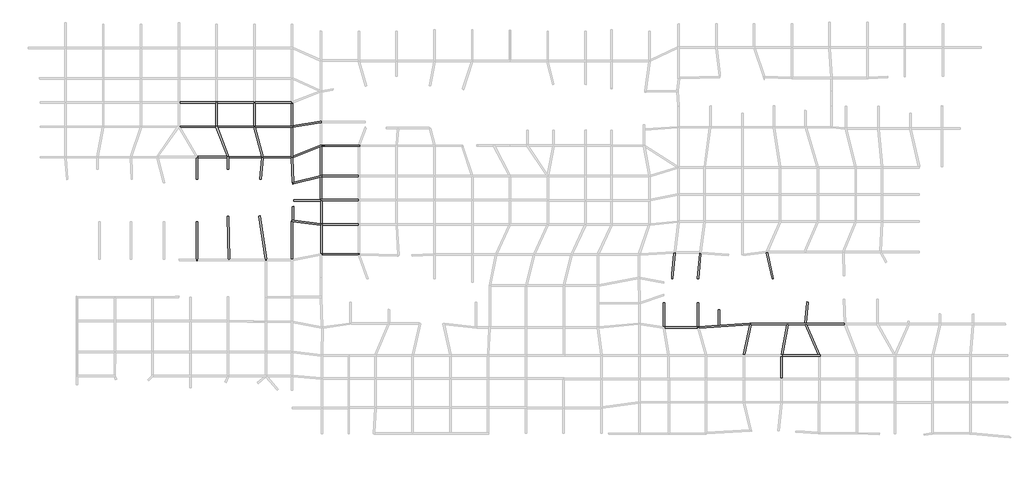
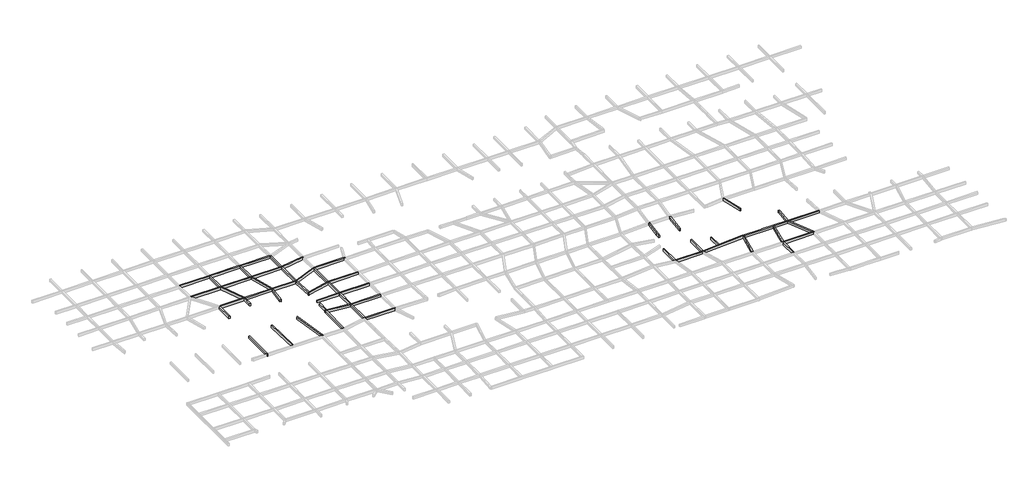
# One storey, part 6 of 15: 53 beams.
"""IFC4 building model written with IfcOpenShell, lengths in millimetres."""

from ifc_helpers import new_model, si_unit, frame, origin, place, context, project, spatial, polyline, outline, extrude, faceted_brep, element, save

model = new_model("IFC4")

# Units and contexts
model_context = context("Model", 3, world=origin())
ifc_project = project(units=[si_unit("LENGTHUNIT", "METRE", prefix="MILLI")], contexts=[model_context])

# Site, building, storey
site = spatial("IfcSite", under=ifc_project)
building = spatial("IfcBuilding", under=site)
storey = spatial("IfcBuildingStorey", under=building, Name="层高", Elevation=3300.0)

# Beams
placement = place(None, origin())
element("IfcBeam", 1, ObjectType="混凝土 - 矩形梁 : KL_beam", at=placement, inside=storey, context=model_context, shape_type="Brep", body=[
    faceted_brep([(153850.3013477, 63968.1790994, 3300.0), (153925.2394262, 63982.5367156, 3300.0), (153925.2394262, 64256.5260367, 3300.0), (153925.2394262, 70092.1684205, 3300.0), (153925.2394262, 70392.1684205, 3300.0), (153625.2394262, 70392.1684205, 3300.0), (153625.2394262, 70122.3059852, 3300.0), (153625.2394262, 64230.5153579, 3300.0), (153793.8501921, 64262.8200114, 3300.0), (153625.2394262, 64230.5153579, 2700.0), (153625.2394262, 70392.1684205, 2700.0), (153625.2394262, 70122.3059852, 2700.0), (153925.2394262, 63982.5367156, 2700.0), (153850.3013477, 63968.1790994, 2700.0), (153793.8501921, 64262.8200114, 2700.0), (153925.2394262, 70392.1684205, 2700.0), (153925.2394262, 70092.1684205, 2700.0), (153925.2394262, 64256.5260367, 2700.0)], [[[0, 1, 2, 3, 4, 5, 6, 7, 8]], [[9, 7, 6, 5, 10, 11]], [[12, 13, 14, 9, 11, 10, 15, 16, 17]], [[1, 12, 17, 16, 15, 4, 3, 2]], [[12, 1, 0, 13]], [[14, 8, 7, 9]], [[8, 14, 13, 0]], [[5, 4, 15, 10]]]),
])
element("IfcBeam", 2, ObjectType="混凝土 - 矩形梁 : KL_beam", at=placement, inside=storey, context=model_context, shape_type="Brep", body=[
    faceted_brep([(153925.2394262, 64256.5260367, 2700.0), (153925.2394262, 64256.5260367, 3300.0), (161350.300938, 64256.5260367, 3300.0), (161650.300938, 64256.5260367, 3300.0), (161650.300938, 64256.5260367, 2700.0), (161350.300938, 64256.5260367, 2700.0), (153925.2394262, 63982.5367156, 2700.0), (153925.2394262, 63982.5367156, 3300.0), (153850.3013477, 63968.1790994, 2700.0), (153850.3013477, 63968.1790994, 3300.0), (153850.3013477, 63956.5260367, 3300.0), (161393.3069779, 63956.5260367, 3300.0), (161497.8826169, 63956.5260367, 3300.0), (161650.300938, 63956.5260367, 3300.0), (161650.300938, 64251.7661343, 3300.0), (161650.300938, 63956.5260367, 2700.0), (153850.3013477, 63956.5260367, 2700.0), (161393.3069779, 63956.5260367, 2700.0), (161497.8826169, 63956.5260367, 2700.0), (161650.300938, 64251.7661343, 2700.0)], [[[0, 1, 2, 3, 4, 5]], [[6, 7, 1, 0]], [[7, 6, 8, 9]], [[1, 7, 9, 10, 11, 12, 13, 14, 3, 2]], [[15, 13, 12, 11, 10, 16, 17, 18]], [[6, 0, 5, 4, 19, 15, 18, 17, 16, 8]], [[9, 8, 16, 10]], [[3, 14, 13, 15, 19, 4]]]),
])
element("IfcBeam", 3, ObjectType="混凝土 - 矩形梁 : KL_beam", at=placement, inside=storey, context=model_context, shape_type="SweptSolid", body=[
    extrude(outline(polyline([(153925.2394262, 70092.1684205), (153925.2394262, 70392.1684205), (161350.300938, 70392.1684205), (161350.300938, 70092.1684205), (153925.2394262, 70092.1684205)])), frame((0.0, 0.0, 2700.0), z_axis=(0.0, 0.0, 1.0), x_axis=(1.0, 0.0, 0.0)), (0.0, 0.0, 1.0), 600.0),
])
element("IfcBeam", 4, ObjectType="混凝土 - 矩形梁 : KL_beam", at=placement, inside=storey, context=model_context, shape_type="Brep", body=[
    faceted_brep([(248649.8189959, 38517.26105, 3300.0), (248949.8189959, 38517.26105, 3300.0), (248949.8189959, 38542.26105, 3300.0), (248949.8189959, 43042.26105, 3300.0), (248649.8189959, 43042.26105, 3300.0), (248949.8189959, 38517.26105, 2700.0), (248949.8189959, 38542.26105, 2700.0), (248949.8189959, 43042.26105, 2700.0), (248649.8189959, 38517.26105, 2700.0), (248649.8189959, 43042.26105, 2700.0)], [[[0, 1, 2, 3, 4]], [[1, 5, 6, 7, 3, 2]], [[5, 8, 9, 7, 6]], [[8, 0, 4, 9]], [[1, 0, 8, 5]], [[4, 3, 7, 9]]]),
])
element("IfcBeam", 5, ObjectType="混凝土 - 矩形梁 : KL_beam", at=placement, inside=storey, context=model_context, shape_type="Brep", body=[
    faceted_brep([(256749.8189959, 43042.26105, 3300.0), (256749.8189959, 43342.26105, 3300.0), (256698.3032407, 43342.26105, 3300.0), (256371.3560571, 43342.26105, 3300.0), (248981.7835465, 43342.26105, 3300.0), (248949.8189959, 43342.26105, 3300.0), (248949.8189959, 43042.26105, 3300.0), (256449.8189959, 43042.26105, 3300.0), (256749.8189959, 43042.26105, 2700.0), (248949.8189959, 43042.26105, 2700.0), (256449.8189959, 43042.26105, 2700.0), (256749.8189959, 43342.26105, 2700.0), (248949.8189959, 43342.26105, 2700.0), (248981.7835465, 43342.26105, 2700.0), (256371.3560571, 43342.26105, 2700.0), (256698.3032407, 43342.26105, 2700.0)], [[[0, 1, 2, 3, 4, 5, 6, 7]], [[8, 0, 7, 6, 9, 10]], [[11, 8, 10, 9, 12, 13, 14, 15]], [[1, 11, 15, 14, 13, 12, 5, 4, 3, 2]], [[6, 5, 12, 9]], [[1, 0, 8, 11]]]),
])
element("IfcBeam", 6, ObjectType="混凝土 - 矩形梁 : KL_beam", at=placement, inside=storey, context=model_context, shape_type="Brep", body=[
    faceted_brep([(261774.3457024, 49601.7141002, 3300.0), (261774.3457024, 49901.7141002, 3300.0), (261720.5296547, 49901.7141002, 3300.0), (253919.7116815, 49901.7141002, 3300.0), (253618.8431569, 49901.7141002, 3300.0), (247159.7341687, 49901.7141002, 3300.0), (247159.7341687, 49841.7141002, 3300.0), (247039.7341687, 49841.7141002, 3300.0), (242265.632488, 49841.7141002, 3300.0), (242214.4093203, 49601.7141002, 3300.0), (242521.1660768, 49601.7141002, 3300.0), (249892.882957, 49601.7141002, 3300.0), (250198.4979655, 49601.7141002, 3300.0), (253659.3709471, 49601.7141002, 3300.0), (253986.3181308, 49601.7141002, 3300.0), (261774.3457024, 49901.7141002, 2700.0), (261774.3457024, 49601.7141002, 2700.0), (253986.3181308, 49601.7141002, 2700.0), (253659.3709471, 49601.7141002, 2700.0), (250198.4979655, 49601.7141002, 2700.0), (249892.882957, 49601.7141002, 2700.0), (242521.1660768, 49601.7141002, 2700.0), (242214.4093203, 49601.7141002, 2700.0), (242265.632488, 49841.7141002, 2700.0), (247159.7341687, 49841.7141002, 2700.0), (247159.7341687, 49901.7141002, 2700.0), (253618.8431569, 49901.7141002, 2700.0), (253919.7116815, 49901.7141002, 2700.0), (261720.5296547, 49901.7141002, 2700.0)], [[[0, 1, 2, 3, 4, 5, 6, 7, 8, 9, 10, 11, 12, 13, 14]], [[15, 16, 17, 18, 19, 20, 21, 22, 23, 24, 25, 26, 27, 28]], [[16, 0, 14, 13, 12, 11, 10, 9, 22, 21, 20, 19, 18, 17]], [[1, 0, 16, 15]], [[22, 9, 8, 23]], [[24, 6, 5, 25]], [[6, 24, 23, 8, 7]], [[1, 15, 28, 27, 26, 25, 5, 4, 3, 2]]]),
])
element("IfcBeam", 7, ObjectType="混凝土 - 矩形梁 : KL_beam", at=placement, inside=storey, context=model_context, shape_type="Brep", body=[
    faceted_brep([(256371.3560571, 43342.26105, 2700.0), (256371.3560571, 43342.26105, 3300.0), (253659.3709471, 49601.7141002, 3300.0), (253659.3709471, 49601.7141002, 2700.0), (256449.8189959, 43342.26105, 2700.0), (256698.3032407, 43342.26105, 2700.0), (256698.3032407, 43342.26105, 3300.0), (256449.8189959, 43342.26105, 3300.0), (253986.3181308, 49601.7141002, 3300.0), (253986.3181308, 49601.7141002, 2700.0)], [[[0, 1, 2, 3]], [[1, 0, 4, 5, 6, 7]], [[7, 6, 8, 2, 1]], [[4, 0, 3, 9, 5]], [[6, 5, 9, 8]], [[3, 2, 8, 9]]]),
])
element("IfcBeam", 8, ObjectType="混凝土 - 矩形梁 : KL_beam", at=placement, inside=storey, context=model_context, shape_type="Brep", body=[
    faceted_brep([(248676.168538, 43342.26105, 3300.0), (248949.8189959, 43342.26105, 3300.0), (248981.7835465, 43342.26105, 3300.0), (250198.4979655, 49601.7141002, 3300.0), (249892.882957, 49601.7141002, 3300.0), (248981.7835465, 43342.26105, 2700.0), (250198.4979655, 49601.7141002, 2700.0), (248949.8189959, 43342.26105, 2700.0), (248676.168538, 43342.26105, 2700.0), (249892.882957, 49601.7141002, 2700.0)], [[[0, 1, 2, 3, 4]], [[2, 5, 6, 3]], [[5, 7, 8, 9, 6]], [[8, 0, 4, 9]], [[0, 8, 7, 5, 2, 1]], [[4, 3, 6, 9]]]),
])
element("IfcBeam", 9, ObjectType="混凝土 - 矩形梁 : KL_beam", at=placement, inside=storey, context=model_context, shape_type="Brep", body=[
    faceted_brep([(253950.2144032, 54253.3773688, 2700.0), (253950.2144032, 54253.3773688, 3300.0), (253964.038385, 54252.3246977, 3300.0), (253964.038385, 54252.3246977, 2700.0), (253950.1342442, 54252.3246977, 2700.0), (253950.1342442, 54252.3246977, 3300.0)], [[[0, 1, 2, 3]], [[0, 3, 4]], [[3, 2, 5, 4]], [[2, 1, 5]], [[1, 0, 4, 5]]]),
    faceted_brep([(253919.7116815, 49901.7141002, 3300.0), (254249.3483857, 54230.5988599, 3300.0), (254109.7167317, 54241.2315565, 3300.0), (254109.7167317, 54132.3246977, 3300.0), (253989.7167317, 54132.3246977, 3300.0), (253940.9964624, 54132.3246977, 3300.0), (253618.8431569, 49901.7141002, 3300.0), (253618.8431569, 49901.7141002, 2700.0), (253940.9964624, 54132.3246977, 2700.0), (254249.3483857, 54230.5988599, 2700.0), (253919.7116815, 49901.7141002, 2700.0), (254109.7167317, 54132.3246977, 2700.0), (254109.7167317, 54241.2315565, 2700.0)], [[[0, 1, 2, 3, 4, 5, 6]], [[7, 6, 5, 8]], [[9, 1, 0, 10]], [[0, 6, 7, 10]], [[11, 3, 2, 12]], [[3, 11, 8, 5, 4]], [[1, 9, 12, 2]], [[9, 10, 7, 8, 11, 12]]]),
])
element("IfcBeam", 10, ObjectType="混凝土 - 矩形梁 : KL_beam", at=placement, inside=storey, context=model_context, shape_type="Brep", body=[
    faceted_brep([(240878.4550975, 43342.26105, 3300.0), (241149.8189959, 43342.26105, 3300.0), (241185.211854, 43342.26105, 3300.0), (242521.1660768, 49601.7141002, 3300.0), (242214.4093203, 49601.7141002, 3300.0), (242211.3807699, 49587.5241911, 3300.0), (241185.211854, 43342.26105, 2700.0), (242521.1660768, 49601.7141002, 2700.0), (241149.8189959, 43342.26105, 2700.0), (240878.4550975, 43342.26105, 2700.0), (242211.3807699, 49587.5241911, 2700.0), (242214.4093203, 49601.7141002, 2700.0)], [[[0, 1, 2, 3, 4, 5]], [[2, 6, 7, 3]], [[6, 8, 9, 10, 11, 7]], [[9, 0, 5, 4, 11, 10]], [[0, 9, 8, 6, 2, 1]], [[4, 3, 7, 11]]]),
])
element("IfcBeam", 11, ObjectType="混凝土 - 矩形梁 : KL_beam", at=placement, inside=storey, context=model_context, shape_type="Brep", body=[
    faceted_brep([(231696.6703608, 48978.5566033, 3300.0), (231696.6703608, 49107.4754781, 3300.0), (231541.189145, 49107.4754781, 3300.0), (231396.6703608, 49107.4754781, 3300.0), (224676.6602363, 49107.4754781, 3300.0), (224538.2100932, 49107.4754781, 3300.0), (224676.6602363, 49086.0272569, 3300.0), (224676.6602363, 48969.2807341, 3300.0), (224702.2876712, 48807.4754781, 3300.0), (231433.6372532, 48807.4754781, 3300.0), (231396.6703608, 48936.3943529, 3300.0), (231433.6372532, 48807.4754781, 2700.0), (224702.2876712, 48807.4754781, 2700.0), (231696.6703608, 49107.4754781, 2700.0), (231696.6703608, 48978.5566033, 2700.0), (231396.6703608, 48936.3943529, 2700.0), (224676.6602363, 48969.2807341, 2700.0), (224676.6602363, 49086.0272569, 2700.0), (224538.2100932, 49107.4754781, 2700.0), (224676.6602363, 49107.4754781, 2700.0), (231396.6703608, 49107.4754781, 2700.0), (231541.189145, 49107.4754781, 2700.0)], [[[0, 1, 2, 3, 4, 5, 6, 7, 8, 9, 10]], [[11, 9, 8, 12]], [[13, 14, 15, 11, 12, 16, 17, 18, 19, 20, 21]], [[1, 13, 21, 20, 19, 18, 5, 4, 3, 2]], [[1, 0, 14, 13]], [[10, 9, 11, 15]], [[8, 7, 16, 12]], [[10, 15, 14, 0]], [[17, 6, 5, 18]], [[6, 17, 16, 7]]]),
])
element("IfcBeam", 12, ObjectType="混凝土 - 矩形梁 : KL_beam", at=placement, inside=storey, context=model_context, shape_type="Brep", body=[
    faceted_brep([(231741.7485438, 48821.3502966, 3300.0), (242211.3807699, 49587.5241911, 3300.0), (242214.4093203, 49601.7141002, 3300.0), (242265.632488, 49841.7141002, 3300.0), (242218.4382799, 49841.7141002, 3300.0), (242218.4382799, 49888.8429011, 3300.0), (236049.8021786, 49437.4184534, 3300.0), (235749.8021786, 49415.4642755, 3300.0), (231696.6703608, 49118.8536857, 3300.0), (231541.189145, 49107.4754781, 3300.0), (231696.6703608, 49107.4754781, 3300.0), (231696.6703608, 48978.5566033, 3300.0), (242211.3807699, 49587.5241911, 2700.0), (231741.7485438, 48821.3502966, 2700.0), (231696.6703608, 48978.5566033, 2700.0), (231696.6703608, 49107.4754781, 2700.0), (231541.189145, 49107.4754781, 2700.0), (231696.6703608, 49118.8536857, 2700.0), (235749.8021786, 49415.4642755, 2700.0), (236049.8021786, 49437.4184534, 2700.0), (242218.4382799, 49888.8429011, 2700.0), (242218.4382799, 49841.7141002, 2700.0), (242265.632488, 49841.7141002, 2700.0), (242214.4093203, 49601.7141002, 2700.0)], [[[0, 1, 2, 3, 4, 5, 6, 7, 8, 9, 10, 11]], [[12, 1, 0, 13]], [[12, 13, 14, 15, 16, 17, 18, 19, 20, 21, 22, 23]], [[16, 9, 8, 7, 6, 5, 20, 19, 18, 17]], [[1, 12, 23, 22, 3, 2]], [[0, 11, 14, 13]], [[15, 10, 9, 16]], [[10, 15, 14, 11]], [[21, 4, 3, 22]], [[4, 21, 20, 5]]]),
])
element("IfcBeam", 13, ObjectType="混凝土 - 矩形梁 : KL_beam", at=placement, inside=storey, context=model_context, shape_type="SweptSolid", body=[
    extrude(outline(polyline([(236049.8021786, 49437.4184534), (235749.8021786, 49415.4642755), (235749.8021786, 52693.0860808), (236049.8021786, 52693.0860808), (236049.8021786, 49437.4184534)])), frame((0.0, 0.0, 2700.0), z_axis=(0.0, 0.0, 1.0), x_axis=(1.0, 0.0, 0.0)), (0.0, 0.0, 1.0), 600.0),
])
element("IfcBeam", 14, ObjectType="混凝土 - 矩形梁 : KL_beam", at=placement, inside=storey, context=model_context, shape_type="SweptSolid", body=[
    extrude(outline(polyline([(231541.189145, 49107.4754781), (231396.6703608, 49107.4754781), (231396.6703608, 54132.3246977), (231696.6703608, 54132.3246977), (231696.6703608, 49118.8536857), (231541.189145, 49107.4754781)])), frame((0.0, 0.0, 2700.0), z_axis=(0.0, 0.0, 1.0), x_axis=(1.0, 0.0, 0.0)), (0.0, 0.0, 1.0), 600.0),
])
element("IfcBeam", 15, ObjectType="混凝土 - 矩形梁 : KL_beam", at=placement, inside=storey, context=model_context, shape_type="SweptSolid", body=[
    extrude(outline(polyline([(224376.6602363, 54091.8381482), (224676.6602363, 54091.8381482), (224676.6602363, 49107.4754781), (224538.2100932, 49107.4754781), (224376.6602363, 49132.5022277), (224376.6602363, 54091.8381482)])), frame((0.0, 0.0, 2700.0), z_axis=(0.0, 0.0, 1.0), x_axis=(1.0, 0.0, 0.0)), (0.0, 0.0, 1.0), 600.0),
])
element("IfcBeam", 16, ObjectType="混凝土 - 矩形梁 : KL_beam", at=placement, inside=storey, context=model_context, shape_type="Brep", body=[
    faceted_brep([(153625.2394262, 75445.2581831, 3300.0), (153625.2394262, 75145.2581831, 3300.0), (153925.2394262, 75145.2581831, 3300.0), (161350.300938, 75145.2581831, 3300.0), (161350.300938, 75445.2581831, 3300.0), (153850.3009381, 75445.2581831, 3300.0), (153625.2394262, 75445.2581831, 2700.0), (161350.300938, 75445.2581831, 2700.0), (153850.3009381, 75445.2581831, 2700.0), (153625.2394262, 75145.2581831, 2700.0), (161350.300938, 75145.2581831, 2700.0), (153925.2394262, 75145.2581831, 2700.0)], [[[0, 1, 2, 3, 4, 5]], [[6, 0, 5, 4, 7, 8]], [[9, 6, 8, 7, 10, 11]], [[1, 9, 11, 10, 3, 2]], [[4, 3, 10, 7]], [[1, 0, 6, 9]]]),
])
element("IfcBeam", 17, ObjectType="混凝土 - 矩形梁 : KL_beam", at=placement, inside=storey, context=model_context, shape_type="Brep", body=[
    faceted_brep([(153625.2394262, 70392.1684205, 3300.0), (153925.2394262, 70392.1684205, 3300.0), (153925.2394262, 75145.2581831, 3300.0), (153625.2394262, 75145.2581831, 3300.0), (153625.2394262, 75142.8652747, 3300.0), (153625.2394262, 75102.1202767, 3300.0), (153625.2394262, 70424.6220705, 3300.0), (153925.2394262, 70392.1684205, 2700.0), (153925.2394262, 75145.2581831, 2700.0), (153625.2394262, 70392.1684205, 2700.0), (153625.2394262, 70424.6220705, 2700.0), (153625.2394262, 75102.1202767, 2700.0), (153625.2394262, 75142.8652747, 2700.0), (153625.2394262, 75145.2581831, 2700.0)], [[[0, 1, 2, 3, 4, 5, 6]], [[1, 7, 8, 2]], [[7, 9, 10, 11, 12, 13, 8]], [[9, 0, 6, 5, 4, 3, 13, 12, 11, 10]], [[1, 0, 9, 7]], [[3, 2, 8, 13]]]),
])
element("IfcBeam", 18, ObjectType="混凝土 - 矩形梁 : KL_beam", at=placement, inside=storey, context=model_context, shape_type="Brep", body=[
    faceted_brep([(139785.4057415, 90592.3894162, 3300.0), (139785.4057415, 90292.3894162, 3300.0), (140096.1315792, 90292.3894162, 3300.0), (147550.2032763, 90292.3894162, 3300.0), (147850.2032763, 90292.3894162, 3300.0), (147850.2032763, 90315.315406, 3300.0), (147850.2032763, 90592.3894162, 3300.0), (147687.7917965, 90592.3894162, 3300.0), (147550.2032763, 90592.3894162, 3300.0), (140050.3009381, 90592.3894162, 3300.0), (139785.4057415, 90292.3894162, 2700.0), (140096.1315792, 90292.3894162, 2700.0), (147550.2032763, 90292.3894162, 2700.0), (147850.2032763, 90292.3894162, 2700.0), (139785.4057415, 90592.3894162, 2700.0), (140050.3009381, 90592.3894162, 2700.0), (147550.2032763, 90592.3894162, 2700.0), (147687.7917965, 90592.3894162, 2700.0), (147850.2032763, 90592.3894162, 2700.0), (147850.2032763, 90315.315406, 2700.0)], [[[0, 1, 2, 3, 4, 5, 6, 7, 8, 9]], [[1, 10, 11, 12, 13, 4, 3, 2]], [[10, 14, 15, 16, 17, 18, 19, 13, 12, 11]], [[14, 0, 9, 8, 7, 6, 18, 17, 16, 15]], [[6, 5, 4, 13, 19, 18]], [[0, 14, 10, 1]]]),
])
element("IfcBeam", 19, ObjectType="混凝土 - 矩形梁 : KL_beam", at=placement, inside=storey, context=model_context, shape_type="Brep", body=[
    faceted_brep([(147550.2032763, 84040.4584193, 3300.0), (147850.2032763, 84040.4584193, 3300.0), (147850.2032763, 84363.1269806, 3300.0), (147850.2032763, 90292.3894162, 3300.0), (147550.2032763, 90292.3894162, 3300.0), (147550.2032763, 84292.3894162, 3300.0), (147550.2032763, 84040.4584193, 2700.0), (147550.2032763, 90292.3894162, 2700.0), (147550.2032763, 84292.3894162, 2700.0), (147850.2032763, 84040.4584193, 2700.0), (147850.2032763, 90292.3894162, 2700.0), (147850.2032763, 84363.1269806, 2700.0)], [[[0, 1, 2, 3, 4, 5]], [[6, 0, 5, 4, 7, 8]], [[9, 6, 8, 7, 10, 11]], [[1, 9, 11, 10, 3, 2]], [[4, 3, 10, 7]], [[1, 0, 6, 9]]]),
])
element("IfcBeam", 20, ObjectType="混凝土 - 矩形梁 : KL_beam", at=placement, inside=storey, context=model_context, shape_type="Brep", body=[
    faceted_brep([(154486.4551572, 86668.5594398, 3300.0), (153850.3009381, 86668.5594398, 3300.0), (153671.6805994, 86668.5594398, 3300.0), (153550.3009381, 86620.4904367, 3300.0), (147850.2032763, 84363.1269806, 3300.0), (147850.2032763, 84040.4584193, 3300.0), (147854.6371658, 84042.2143366, 3300.0), (153550.3009381, 86297.8218754, 3300.0), (153728.9212768, 86368.5594398, 3300.0), (153671.6805994, 86668.5594398, 2700.0), (153550.3009381, 86620.4904367, 2700.0), (147850.2032763, 84363.1269806, 2700.0), (153850.3009381, 86668.5594398, 2700.0), (154486.4551572, 86668.5594398, 2700.0), (153728.9212768, 86368.5594398, 2700.0), (153550.3009381, 86297.8218754, 2700.0), (147854.6371658, 84042.2143366, 2700.0), (147850.2032763, 84040.4584193, 2700.0)], [[[0, 1, 2, 3, 4, 5, 6, 7, 8]], [[2, 9, 10, 11, 4, 3]], [[9, 12, 13, 14, 15, 16, 17, 11, 10]], [[13, 0, 8, 7, 6, 5, 17, 16, 15, 14]], [[5, 4, 11, 17]], [[2, 1, 0, 13, 12, 9]]]),
])
element("IfcBeam", 21, ObjectType="混凝土 - 矩形梁 : KL_beam", at=placement, inside=storey, context=model_context, shape_type="Brep", body=[
    faceted_brep([(141404.1146306, 84292.3894162, 3300.0), (141448.0146947, 84129.6668995, 3300.0), (141485.0500751, 83992.3894162, 3300.0), (141736.1368385, 83992.3894162, 3300.0), (147556.4981693, 83992.3894162, 3300.0), (147856.7739124, 83992.3894162, 3300.0), (147854.6371658, 84042.2143366, 3300.0), (147850.2032763, 84040.4584193, 3300.0), (147550.2032763, 84040.4584193, 3300.0), (147550.2032763, 84244.3204132, 3300.0), (147550.2032763, 84292.3894162, 3300.0), (141714.8404682, 84292.3894162, 3300.0), (147856.7739124, 83992.3894162, 2700.0), (141485.0500751, 83992.3894162, 2700.0), (141736.1368385, 83992.3894162, 2700.0), (147556.4981693, 83992.3894162, 2700.0), (141448.0146947, 84129.6668995, 2700.0), (141404.1146306, 84292.3894162, 2700.0), (141714.8404682, 84292.3894162, 2700.0), (147550.2032763, 84292.3894162, 2700.0), (147550.2032763, 84244.3204132, 2700.0), (147550.2032763, 84040.4584193, 2700.0), (147850.2032763, 84040.4584193, 2700.0), (147854.6371658, 84042.2143366, 2700.0)], [[[0, 1, 2, 3, 4, 5, 6, 7, 8, 9, 10, 11]], [[12, 5, 4, 3, 2, 13, 14, 15]], [[13, 16, 17, 18, 19, 20, 21, 22, 23, 12, 15, 14]], [[10, 19, 18, 17, 0, 11]], [[5, 12, 23, 6]], [[19, 10, 9, 8, 21, 20]], [[2, 1, 0, 17, 16, 13]], [[21, 8, 7, 22]], [[7, 6, 23, 22]]]),
])
element("IfcBeam", 22, ObjectType="混凝土 - 矩形梁 : KL_beam", at=placement, inside=storey, context=model_context, shape_type="SweptSolid", body=[
    extrude(outline(polyline([(139785.4057415, 90292.3894162), (140096.1315792, 90292.3894162), (141714.8404682, 84292.3894162), (141404.1146306, 84292.3894162), (139785.4057415, 90292.3894162)])), frame((0.0, 0.0, 2700.0), z_axis=(0.0, 0.0, 1.0), x_axis=(1.0, 0.0, 0.0)), (0.0, 0.0, 1.0), 600.0),
])
element("IfcBeam", 23, ObjectType="混凝土 - 矩形梁 : KL_beam", at=placement, inside=storey, context=model_context, shape_type="Brep", body=[
    faceted_brep([(153777.0075912, 80408.9310909, 3300.0), (153681.6957031, 80384.9176514, 3300.0), (153550.3009381, 80351.813279, 3300.0), (148072.0909243, 78971.6007231, 3300.0), (147870.12079, 78920.7151757, 3300.0), (147870.12079, 78841.1444171, 3300.0), (147990.12079, 78841.1444171, 3300.0), (147990.12079, 78641.5736585, 3300.0), (153550.3009381, 80042.4382536, 3300.0), (153850.3009381, 80118.0220238, 3300.0), (153783.0576788, 80384.9176514, 3300.0), (153777.0075912, 80408.9310909, 2700.0), (153681.6957031, 80384.9176514, 2700.0), (153550.3009381, 80351.813279, 2700.0), (148072.0909243, 78971.6007231, 2700.0), (147870.12079, 78920.7151757, 2700.0), (153783.0576788, 80384.9176514, 2700.0), (153850.3009381, 80118.0220238, 2700.0), (153550.3009381, 80042.4382536, 2700.0), (147990.12079, 78641.5736585, 2700.0), (147990.12079, 78841.1444171, 2700.0), (147870.12079, 78841.1444171, 2700.0)], [[[0, 1, 2, 3, 4, 5, 6, 7, 8, 9, 10]], [[4, 3, 2, 1, 0, 11, 12, 13, 14, 15]], [[15, 14, 13, 12, 11, 16, 17, 18, 19, 20, 21]], [[17, 9, 8, 7, 19, 18]], [[4, 15, 21, 5]], [[20, 6, 5, 21]], [[6, 20, 19, 7]], [[9, 17, 16, 11, 0, 10]]]),
])
element("IfcBeam", 24, ObjectType="混凝土 - 矩形梁 : KL_beam", at=placement, inside=storey, context=model_context, shape_type="SweptSolid", body=[
    extrude(outline(polyline([(147788.1506557, 78590.6881111), (147782.5560243, 78721.1444171), (147870.12079, 78721.1444171), (147870.12079, 78611.3401504), (147788.1506557, 78590.6881111)])), frame((0.0, 0.0, 2700.0), z_axis=(0.0, 0.0, 1.0), x_axis=(1.0, 0.0, 0.0)), (0.0, 0.0, 1.0), 600.0),
    extrude(outline(polyline([(147777.4098126, 78841.1444171), (147556.4981693, 83992.3894162), (147856.7739124, 83992.3894162), (148072.0909243, 78971.6007231), (147870.12079, 78920.7151757), (147870.12079, 78841.1444171), (147777.4098126, 78841.1444171)])), frame((0.0, 0.0, 2700.0), z_axis=(0.0, 0.0, 1.0), x_axis=(1.0, 0.0, 0.0)), (0.0, 0.0, 1.0), 600.0),
])
element("IfcBeam", 25, ObjectType="混凝土 - 矩形梁 : KL_beam", at=placement, inside=storey, context=model_context, shape_type="Brep", body=[
    faceted_brep([(141013.7858677, 79640.2608397, 3300.0), (141310.12079, 79640.2608397, 3300.0), (141310.12079, 79587.8936497, 3300.0), (141736.1368385, 83992.3894162, 3300.0), (141485.0500751, 83992.3894162, 3300.0), (141448.0146947, 84129.6668995, 3300.0), (141434.7368045, 83992.3894162, 3300.0), (141013.7858677, 79640.2608397, 2700.0), (141448.0146947, 84129.6668995, 2700.0), (141434.7368045, 83992.3894162, 2700.0), (141310.12079, 79640.2608397, 2700.0), (141485.0500751, 83992.3894162, 2700.0), (141736.1368385, 83992.3894162, 2700.0), (141310.12079, 79587.8936497, 2700.0)], [[[0, 1, 2, 3, 4, 5, 6]], [[7, 0, 6, 5, 8, 9]], [[10, 7, 9, 8, 11, 12, 13]], [[2, 13, 12, 3]], [[10, 1, 0, 7]], [[1, 10, 13, 2]], [[11, 4, 3, 12]], [[4, 11, 8, 5]]]),
])
element("IfcBeam", 26, ObjectType="混凝土 - 矩形梁 : KL_beam", at=placement, inside=storey, context=model_context, shape_type="Brep", body=[
    faceted_brep([(134650.2032763, 84292.3894162, 3300.0), (134603.29542, 84292.3894162, 3300.0), (134350.2032763, 84292.3894162, 3300.0), (134350.2032763, 84114.5885595, 3300.0), (134350.2032763, 84017.4440548, 3300.0), (134350.2032763, 81642.3565617, 3300.0), (134650.2032763, 81642.3565617, 3300.0), (134650.2032763, 83992.3894162, 3300.0), (134350.2032763, 84292.3894162, 2700.0), (134350.2032763, 84114.5885595, 2700.0), (134350.2032763, 84017.4440548, 2700.0), (134350.2032763, 81642.3565617, 2700.0), (134603.29542, 84292.3894162, 2700.0), (134650.2032763, 84292.3894162, 2700.0), (134650.2032763, 83992.3894162, 2700.0), (134650.2032763, 81642.3565617, 2700.0)], [[[0, 1, 2, 3, 4, 5, 6, 7]], [[2, 8, 9, 10, 11, 5, 4, 3]], [[8, 12, 13, 14, 15, 11, 10, 9]], [[13, 0, 7, 6, 15, 14]], [[6, 5, 11, 15]], [[2, 1, 0, 13, 12, 8]]]),
])
element("IfcBeam", 27, ObjectType="混凝土 - 矩形梁 : KL_beam", at=placement, inside=storey, context=model_context, shape_type="SweptSolid", body=[
    extrude(outline(polyline([(141404.1146306, 84292.3894162), (141448.0146947, 84129.6668995), (141434.7368045, 83992.3894162), (134650.2032763, 83992.3894162), (134650.2032763, 84292.3894162), (141404.1146306, 84292.3894162)])), frame((0.0, 0.0, 2700.0), z_axis=(0.0, 0.0, 1.0), x_axis=(1.0, 0.0, 0.0)), (0.0, 0.0, 1.0), 600.0),
])
element("IfcBeam", 28, ObjectType="混凝土 - 矩形梁 : KL_beam", at=placement, inside=storey, context=model_context, shape_type="Brep", body=[
    faceted_brep([(134350.2032763, 84114.5885595, 3300.0), (134350.2032763, 84292.3894162, 3300.0), (134603.29542, 84292.3894162, 3300.0), (132300.1112098, 90292.3894162, 3300.0), (132184.9519993, 90592.3894162, 3300.0), (131950.3009381, 90592.3894162, 3300.0), (131863.6085012, 90592.3894162, 3300.0), (131978.7677117, 90292.3894162, 3300.0), (134272.3343473, 84317.4440548, 3300.0), (134603.29542, 84292.3894162, 2700.0), (132300.1112098, 90292.3894162, 2700.0), (132184.9519993, 90592.3894162, 2700.0), (134350.2032763, 84292.3894162, 2700.0), (134350.2032763, 84114.5885595, 2700.0), (134272.3343473, 84317.4440548, 2700.0), (131978.7677117, 90292.3894162, 2700.0), (131863.6085012, 90592.3894162, 2700.0), (131950.3009381, 90592.3894162, 2700.0)], [[[0, 1, 2, 3, 4, 5, 6, 7, 8]], [[2, 9, 10, 11, 4, 3]], [[12, 13, 14, 15, 16, 17, 11, 10, 9]], [[13, 0, 8, 7, 6, 16, 15, 14]], [[12, 1, 0, 13]], [[1, 12, 9, 2]], [[6, 5, 4, 11, 17, 16]]]),
])
element("IfcBeam", 29, ObjectType="混凝土 - 矩形梁 : KL_beam", at=placement, inside=storey, context=model_context, shape_type="Brep", body=[
    faceted_brep([(128220.534006, 84209.0427364, 3300.0), (128220.534006, 84317.4440548, 3300.0), (128155.3999228, 84317.4440548, 3300.0), (128220.534006, 84317.4440548, 2700.0), (128220.534006, 84209.0427364, 2700.0), (128155.3999228, 84317.4440548, 2700.0)], [[[0, 1, 2]], [[3, 4, 5]], [[1, 0, 4, 3]], [[5, 2, 1, 3]], [[0, 2, 5, 4]]]),
    faceted_brep([(127920.534006, 79640.2608397, 2700.0), (127920.534006, 79640.2608397, 3300.0), (127920.534006, 84017.4440548, 3300.0), (127920.534006, 84017.4440548, 2700.0), (128220.534006, 79640.2608397, 3300.0), (128220.534006, 79640.2608397, 2700.0), (127985.6680893, 84017.4440548, 3300.0), (127985.6680893, 84017.4440548, 2700.0), (128220.534006, 84158.5657349, 3300.0), (128220.534006, 84158.5657349, 2700.0), (128220.534006, 84017.4440548, 3300.0), (128220.534006, 84017.4440548, 2700.0)], [[[0, 1, 2, 3]], [[4, 1, 0, 5]], [[3, 2, 6, 7]], [[6, 8, 9, 7]], [[1, 4, 10, 8, 6, 2]], [[5, 0, 3, 7, 9, 11]], [[4, 5, 11, 9, 8, 10]]]),
])
element("IfcBeam", 30, ObjectType="混凝土 - 矩形梁 : KL_beam", at=placement, inside=storey, context=model_context, shape_type="SweptSolid", body=[
    extrude(outline(polyline([(128220.534006, 84158.5657349), (128242.8182795, 84171.9554773), (128220.534006, 84209.0427364), (128220.534006, 84317.4440548), (134272.3343473, 84317.4440548), (134350.2032763, 84114.5885595), (134350.2032763, 84017.4440548), (128220.534006, 84017.4440548), (128220.534006, 84158.5657349)])), frame((0.0, 0.0, 2700.0), z_axis=(0.0, 0.0, 1.0), x_axis=(1.0, 0.0, 0.0)), (0.0, 0.0, 1.0), 600.0),
])
element("IfcBeam", 31, ObjectType="混凝土 - 矩形梁 : KL_beam", at=placement, inside=storey, context=model_context, shape_type="SweptSolid", body=[
    extrude(outline(polyline([(124565.2905543, 90292.3894162), (124450.1664518, 90483.9880978), (124450.1664518, 90592.3894162), (131863.6085012, 90592.3894162), (131978.7677117, 90292.3894162), (124565.2905543, 90292.3894162)])), frame((0.0, 0.0, 2700.0), z_axis=(0.0, 0.0, 1.0), x_axis=(1.0, 0.0, 0.0)), (0.0, 0.0, 1.0), 600.0),
])
element("IfcBeam", 32, ObjectType="混凝土 - 矩形梁 : KL_beam", at=placement, inside=storey, context=model_context, shape_type="Brep", body=[
    faceted_brep([(139785.4057415, 90292.3894162, 3300.0), (139785.4057415, 90592.3894162, 3300.0), (139750.3009381, 90592.3894162, 3300.0), (132250.3009381, 90592.3894162, 3300.0), (132184.9519993, 90592.3894162, 3300.0), (132300.1112098, 90292.3894162, 3300.0), (139785.4057415, 90292.3894162, 2700.0), (132300.1112098, 90292.3894162, 2700.0), (139785.4057415, 90592.3894162, 2700.0), (132184.9519993, 90592.3894162, 2700.0), (132250.3009381, 90592.3894162, 2700.0), (139750.3009381, 90592.3894162, 2700.0)], [[[0, 1, 2, 3, 4, 5]], [[6, 0, 5, 7]], [[8, 6, 7, 9, 10, 11]], [[1, 8, 11, 10, 9, 4, 3, 2]], [[1, 0, 6, 8]], [[5, 4, 9, 7]]]),
])
element("IfcBeam", 33, ObjectType="混凝土 - 矩形梁 : KL_beam", at=placement, inside=storey, context=model_context, shape_type="Brep", body=[
    faceted_brep([(131950.3009381, 90592.3894162, 3300.0), (132184.9519993, 90592.3894162, 3300.0), (132250.3009381, 90592.3894162, 3300.0), (132250.3009381, 95292.1233035, 3300.0), (132250.3009381, 95592.1233035, 3300.0), (131950.3009381, 95592.1233035, 3300.0), (131950.3009381, 95292.1233035, 3300.0), (131950.3009381, 90592.3894162, 2700.0), (131950.3009381, 95592.1233035, 2700.0), (131950.3009381, 95292.1233035, 2700.0), (132250.3009381, 90592.3894162, 2700.0), (132184.9519993, 90592.3894162, 2700.0), (132250.3009381, 95592.1233035, 2700.0), (132250.3009381, 95292.1233035, 2700.0)], [[[0, 1, 2, 3, 4, 5, 6]], [[7, 0, 6, 5, 8, 9]], [[10, 11, 7, 9, 8, 12, 13]], [[2, 10, 13, 12, 4, 3]], [[0, 7, 11, 10, 2, 1]], [[5, 4, 12, 8]]]),
])
element("IfcBeam", 34, ObjectType="混凝土 - 矩形梁 : KL_beam", at=placement, inside=storey, context=model_context, shape_type="Brep", body=[
    faceted_brep([(147687.7917965, 90592.3894162, 3300.0), (147850.2032763, 90619.4515862, 3300.0), (153550.3009381, 91569.2428953, 3300.0), (153687.8894584, 91592.168885, 3300.0), (153687.8894584, 91592.168885, 2700.0), (153550.3009381, 91569.2428953, 2700.0), (147850.2032763, 90619.4515862, 2700.0), (147687.7917965, 90592.3894162, 2700.0), (147850.2032763, 90592.3894162, 2700.0), (147850.2032763, 90592.3894162, 3300.0), (147850.2032763, 90315.315406, 2700.0), (147850.2032763, 90315.315406, 3300.0), (153550.3009381, 91265.106715, 3300.0), (153712.7124179, 91292.168885, 3300.0), (153712.7124179, 91292.168885, 2700.0), (153550.3009381, 91265.106715, 2700.0)], [[[0, 1, 2, 3, 4, 5, 6, 7]], [[8, 9, 0, 7]], [[9, 8, 10, 11]], [[11, 12, 13, 3, 2, 1, 0, 9]], [[7, 6, 5, 4, 14, 15, 10, 8]], [[13, 12, 11, 10, 15, 14]], [[13, 14, 4, 3]]]),
])
element("IfcBeam", 35, ObjectType="混凝土 - 矩形梁 : KL_beam", at=placement, inside=storey, context=model_context, shape_type="Brep", body=[
    faceted_brep([(153850.3009381, 75445.2581831, 3300.0), (153850.3009381, 80084.9176514, 3300.0), (153850.3009381, 80118.0220238, 3300.0), (153550.3009381, 80042.4382536, 3300.0), (153550.3009381, 75402.1202767, 3300.0), (153550.3009381, 75142.8652747, 3300.0), (153625.2394262, 75142.8652747, 3300.0), (153625.2394262, 75145.2581831, 3300.0), (153625.2394262, 75445.2581831, 3300.0), (153550.3009381, 75142.8652747, 2700.0), (153550.3009381, 80042.4382536, 2700.0), (153550.3009381, 75402.1202767, 2700.0), (153850.3009381, 80118.0220238, 2700.0), (153850.3009381, 80084.9176514, 2700.0), (153850.3009381, 75445.2581831, 2700.0), (153625.2394262, 75445.2581831, 2700.0), (153625.2394262, 75145.2581831, 2700.0), (153625.2394262, 75142.8652747, 2700.0)], [[[0, 1, 2, 3, 4, 5, 6, 7, 8]], [[9, 5, 4, 3, 10, 11]], [[12, 13, 14, 15, 16, 17, 9, 11, 10]], [[2, 1, 0, 14, 13, 12]], [[5, 9, 17, 6]], [[8, 15, 14, 0]], [[15, 8, 7, 6, 17, 16]], [[3, 2, 12, 10]]]),
])
element("IfcBeam", 36, ObjectType="混凝土 - 矩形梁 : KL_beam", at=placement, inside=storey, context=model_context, shape_type="SweptSolid", body=[
    extrude(outline(polyline([(147990.12079, 75102.1202767), (147990.12079, 75402.1202767), (153550.3009381, 75402.1202767), (153550.3009381, 75142.8652747), (153625.2394262, 75142.8652747), (153625.2394262, 75102.1202767), (147990.12079, 75102.1202767)])), frame((0.0, 0.0, 2700.0), z_axis=(0.0, 0.0, 1.0), x_axis=(1.0, 0.0, 0.0)), (0.0, 0.0, 1.0), 600.0),
])
element("IfcBeam", 37, ObjectType="混凝土 - 矩形梁 : KL_beam", at=placement, inside=storey, context=model_context, shape_type="Brep", body=[
    faceted_brep([(147550.2032763, 70878.6460655, 3300.0), (147850.2032763, 70841.2961603, 3300.0), (153625.2394262, 70122.3059852, 3300.0), (153625.2394262, 70392.1684205, 3300.0), (153625.2394262, 70424.6220705, 3300.0), (148080.12079, 71114.9875878, 3300.0), (147780.12079, 71152.337493, 3300.0), (147587.2670386, 71176.3477241, 3300.0), (153625.2394262, 70424.6220705, 2700.0), (148080.12079, 71114.9875878, 2700.0), (147780.12079, 71152.337493, 2700.0), (147587.2670386, 71176.3477241, 2700.0), (153625.2394262, 70392.1684205, 2700.0), (153625.2394262, 70122.3059852, 2700.0), (147850.2032763, 70841.2961603, 2700.0), (147550.2032763, 70878.6460655, 2700.0)], [[[0, 1, 2, 3, 4, 5, 6, 7]], [[7, 6, 5, 4, 8, 9, 10, 11]], [[11, 10, 9, 8, 12, 13, 14, 15]], [[2, 1, 0, 15, 14, 13]], [[8, 4, 3, 2, 13, 12]], [[0, 7, 11, 15]]]),
])
element("IfcBeam", 38, ObjectType="混凝土 - 矩形梁 : KL_beam", at=placement, inside=storey, context=model_context, shape_type="Brep", body=[
    faceted_brep([(147990.12079, 73932.1202767, 3300.0), (147870.12079, 73932.1202767, 3300.0), (147780.12079, 73932.1202767, 3300.0), (147780.12079, 71152.337493, 3300.0), (148080.12079, 71114.9875878, 3300.0), (148080.12079, 74052.1202767, 3300.0), (147990.12079, 74052.1202767, 3300.0), (147780.12079, 73932.1202767, 2700.0), (147780.12079, 71152.337493, 2700.0), (147990.12079, 73932.1202767, 2700.0), (147990.12079, 74052.1202767, 2700.0), (148080.12079, 74052.1202767, 2700.0), (148080.12079, 71114.9875878, 2700.0)], [[[0, 1, 2, 3, 4, 5, 6]], [[2, 7, 8, 3]], [[7, 9, 10, 11, 12, 8]], [[11, 5, 4, 12]], [[5, 11, 10, 6]], [[0, 9, 7, 2, 1]], [[4, 3, 8, 12]], [[9, 0, 6, 10]]]),
])
element("IfcBeam", 39, ObjectType="混凝土 - 矩形梁 : KL_beam", at=placement, inside=storey, context=model_context, shape_type="Brep", body=[
    faceted_brep([(147550.2032763, 70878.6460655, 3300.0), (147550.2032763, 63092.591237, 3300.0), (147550.2032763, 63066.5805586, 3300.0), (147850.2032763, 63124.0584782, 3300.0), (147850.2032763, 70841.2961603, 3300.0), (147850.2032763, 63124.0584782, 2700.0), (147850.2032763, 70841.2961603, 2700.0), (147550.2032763, 63066.5805586, 2700.0), (147550.2032763, 63092.591237, 2700.0), (147550.2032763, 70878.6460655, 2700.0)], [[[0, 1, 2, 3, 4]], [[3, 5, 6, 4]], [[7, 8, 9, 6, 5]], [[2, 1, 0, 9, 8, 7]], [[3, 2, 7, 5]], [[0, 4, 6, 9]]]),
])
element("IfcBeam", 40, ObjectType="混凝土 - 矩形梁 : KL_beam", at=placement, inside=storey, context=model_context, shape_type="Brep", body=[
    faceted_brep([(141092.8747325, 72052.4548583, 3300.0), (141010.165529, 72052.4548583, 3300.0), (141010.165529, 71932.4548583, 3300.0), (140807.4563255, 71932.4548583, 3300.0), (142126.1667579, 63092.591237, 3300.0), (142170.9200648, 62792.591237, 3300.0), (142450.2032763, 62792.591237, 3300.0), (142474.2397946, 62792.591237, 3300.0), (142429.4864877, 63092.591237, 3300.0), (141092.8747325, 72052.4548583, 2700.0), (142474.2397946, 62792.591237, 2700.0), (142429.4864877, 63092.591237, 2700.0), (141010.165529, 72052.4548583, 2700.0), (142450.2032763, 62792.591237, 2700.0), (142170.9200648, 62792.591237, 2700.0), (142126.1667579, 63092.591237, 2700.0), (140807.4563255, 71932.4548583, 2700.0), (141010.165529, 71932.4548583, 2700.0)], [[[0, 1, 2, 3, 4, 5, 6, 7, 8]], [[9, 0, 8, 7, 10, 11]], [[12, 9, 11, 10, 13, 14, 15, 16, 17]], [[14, 5, 4, 3, 16, 15]], [[0, 9, 12, 1]], [[17, 2, 1, 12]], [[2, 17, 16, 3]], [[7, 6, 5, 14, 13, 10]]]),
])
element("IfcBeam", 41, ObjectType="混凝土 - 矩形梁 : KL_beam", at=placement, inside=storey, context=model_context, shape_type="Brep", body=[
    faceted_brep([(134550.2390825, 62939.313735, 3300.0), (134550.2390825, 62939.313735, 2700.0), (134850.1658492, 62945.9420507, 2700.0), (134850.1658492, 62945.9420507, 3300.0), (134846.9249344, 63092.591237, 3300.0), (134651.5658886, 71932.4548583, 3300.0), (134351.4926375, 71932.4548583, 3300.0), (134546.8516833, 63092.591237, 3300.0), (134846.9249344, 63092.591237, 2700.0), (134651.5658886, 71932.4548583, 2700.0), (134546.8516833, 63092.591237, 2700.0), (134351.4926375, 71932.4548583, 2700.0)], [[[0, 1, 2, 3]], [[0, 3, 4, 5, 6, 7]], [[3, 2, 8, 9, 5, 4]], [[2, 1, 10, 11, 9, 8]], [[1, 0, 7, 6, 11, 10]], [[6, 5, 9, 11]]]),
])
element("IfcBeam", 42, ObjectType="混凝土 - 矩形梁 : KL_beam", at=placement, inside=storey, context=model_context, shape_type="Brep", body=[
    faceted_brep([(127950.8470615, 62792.591237, 3300.0), (128250.8470615, 62792.591237, 3300.0), (128250.8470615, 63092.591237, 3300.0), (128250.8470615, 70832.1232979, 3300.0), (127950.8470615, 70832.1232979, 3300.0), (127950.8470615, 63092.591237, 3300.0), (128250.8470615, 62792.591237, 2700.0), (128250.8470615, 63092.591237, 2700.0), (128250.8470615, 70832.1232979, 2700.0), (127950.8470615, 62792.591237, 2700.0), (127950.8470615, 63092.591237, 2700.0), (127950.8470615, 70832.1232979, 2700.0)], [[[0, 1, 2, 3, 4, 5]], [[1, 6, 7, 8, 3, 2]], [[6, 9, 10, 11, 8, 7]], [[9, 0, 5, 4, 11, 10]], [[4, 3, 8, 11]], [[1, 0, 9, 6]]]),
])
element("IfcBeam", 43, ObjectType="混凝土 - 矩形梁 : KL_beam", at=placement, inside=storey, context=model_context, shape_type="Brep", body=[
    faceted_brep([(161650.300938, 86368.5594398, 3300.0), (161650.300938, 86668.5594398, 3300.0), (161397.2087943, 86668.5594398, 3300.0), (154486.4551572, 86668.5594398, 3300.0), (153728.9212768, 86368.5594398, 3300.0), (153850.3009381, 86368.5594398, 3300.0), (161350.300938, 86368.5594398, 3300.0), (161650.300938, 86368.5594398, 2700.0), (153728.9212768, 86368.5594398, 2700.0), (153850.3009381, 86368.5594398, 2700.0), (161350.300938, 86368.5594398, 2700.0), (161650.300938, 86668.5594398, 2700.0), (154486.4551572, 86668.5594398, 2700.0), (161397.2087943, 86668.5594398, 2700.0)], [[[0, 1, 2, 3, 4, 5, 6]], [[7, 0, 6, 5, 4, 8, 9, 10]], [[11, 7, 10, 9, 8, 12, 13]], [[1, 11, 13, 12, 3, 2]], [[4, 3, 12, 8]], [[1, 0, 7, 11]]]),
])
element("IfcBeam", 44, ObjectType="混凝土 - 矩形梁 : KL_beam", at=placement, inside=storey, context=model_context, shape_type="Brep", body=[
    faceted_brep([(153681.6957031, 80384.9176514, 3300.0), (153550.3009381, 80384.9176514, 3300.0), (153550.3009381, 80351.813279, 3300.0), (153550.3009381, 80384.9176514, 2700.0), (153681.6957031, 80384.9176514, 2700.0), (153550.3009381, 80351.813279, 2700.0)], [[[0, 1, 2]], [[3, 4, 5]], [[1, 0, 4, 3]], [[5, 2, 1, 3]], [[0, 2, 5, 4]]]),
    faceted_brep([(161350.300938, 80084.9176514, 2700.0), (161350.300938, 80084.9176514, 3300.0), (153850.3009381, 80084.9176514, 3300.0), (153850.3009381, 80084.9176514, 2700.0), (161350.300938, 80384.9176514, 3300.0), (161350.300938, 80384.9176514, 2700.0), (153850.3009381, 80118.0220238, 3300.0), (153783.0576788, 80384.9176514, 3300.0), (153783.0576788, 80384.9176514, 2700.0), (153850.3009381, 80118.0220238, 2700.0), (153850.3009381, 80384.9176514, 3300.0), (153850.3009381, 80384.9176514, 2700.0)], [[[0, 1, 2, 3]], [[4, 1, 0, 5]], [[6, 7, 8, 9]], [[3, 2, 6, 9]], [[1, 4, 10, 7, 6, 2]], [[5, 0, 3, 9, 8, 11]], [[4, 5, 11, 8, 7, 10]]]),
])
element("IfcBeam", 45, ObjectType="混凝土 - 矩形梁 : KL_beam", at=placement, inside=storey, context=model_context, shape_type="SweptSolid", body=[
    extrude(outline(polyline([(153550.3009381, 86297.8218754), (153728.9212768, 86368.5594398), (153850.3009381, 86368.5594398), (153850.3009381, 80384.9176514), (153783.0576788, 80384.9176514), (153777.0075912, 80408.9310909), (153681.6957031, 80384.9176514), (153550.3009381, 80384.9176514), (153550.3009381, 86297.8218754)])), frame((0.0, 0.0, 2700.0), z_axis=(0.0, 0.0, 1.0), x_axis=(1.0, 0.0, 0.0)), (0.0, 0.0, 1.0), 600.0),
])
element("IfcBeam", 46, ObjectType="混凝土 - 矩形梁 : KL_beam", at=placement, inside=storey, context=model_context, shape_type="SweptSolid", body=[
    extrude(outline(polyline([(124450.1664518, 95292.1233035), (124450.1664518, 95592.1233035), (131950.3009381, 95592.1233035), (131950.3009381, 95292.1233035), (124450.1664518, 95292.1233035)])), frame((0.0, 0.0, 2700.0), z_axis=(0.0, 0.0, 1.0), x_axis=(1.0, 0.0, 0.0)), (0.0, 0.0, 1.0), 600.0),
])
element("IfcBeam", 47, ObjectType="混凝土 - 矩形梁 : KL_beam", at=placement, inside=storey, context=model_context, shape_type="SweptSolid", body=[
    extrude(outline(polyline([(139750.3009381, 95592.1233035), (139750.3009381, 95292.1233035), (132250.3009381, 95292.1233035), (132250.3009381, 95592.1233035), (139750.3009381, 95592.1233035)])), frame((0.0, 0.0, 2700.0), z_axis=(0.0, 0.0, 1.0), x_axis=(1.0, 0.0, 0.0)), (0.0, 0.0, 1.0), 600.0),
])
element("IfcBeam", 48, ObjectType="混凝土 - 矩形梁 : KL_beam", at=placement, inside=storey, context=model_context, shape_type="Brep", body=[
    faceted_brep([(147850.2032763, 95292.1233035, 3300.0), (147850.2032763, 95338.9797898, 3300.0), (147550.2032763, 95338.9797898, 3300.0), (147550.2032763, 95545.2668173, 3300.0), (147550.2032763, 95592.1233035, 3300.0), (140050.3009381, 95592.1233035, 3300.0), (140050.3009381, 95292.1233035, 3300.0), (147550.2032763, 95292.1233035, 3300.0), (147850.2032763, 95292.1233035, 2700.0), (140050.3009381, 95292.1233035, 2700.0), (147550.2032763, 95292.1233035, 2700.0), (147850.2032763, 95338.9797898, 2700.0), (140050.3009381, 95592.1233035, 2700.0), (147550.2032763, 95592.1233035, 2700.0), (147550.2032763, 95545.2668173, 2700.0), (147550.2032763, 95338.9797898, 2700.0)], [[[0, 1, 2, 3, 4, 5, 6, 7]], [[8, 0, 7, 6, 9, 10]], [[11, 8, 10, 9, 12, 13, 14, 15]], [[4, 13, 12, 5]], [[0, 8, 11, 1]], [[13, 4, 3, 2, 15, 14]], [[6, 5, 12, 9]], [[15, 2, 1, 11]]]),
])
element("IfcBeam", 49, ObjectType="混凝土 - 矩形梁 : KL_beam", at=placement, inside=storey, context=model_context, shape_type="Brep", body=[
    faceted_brep([(139750.3009381, 90592.3894162, 3300.0), (139785.4057415, 90592.3894162, 3300.0), (140050.3009381, 90592.3894162, 3300.0), (140050.3009381, 95292.1233035, 3300.0), (139750.3009381, 95292.1233035, 3300.0), (139750.3009381, 90592.3894162, 2700.0), (139750.3009381, 95292.1233035, 2700.0), (140050.3009381, 90592.3894162, 2700.0), (139785.4057415, 90592.3894162, 2700.0), (140050.3009381, 95292.1233035, 2700.0)], [[[0, 1, 2, 3, 4]], [[5, 0, 4, 6]], [[7, 8, 5, 6, 9]], [[2, 7, 9, 3]], [[7, 2, 1, 0, 5, 8]], [[4, 3, 9, 6]]]),
])
element("IfcBeam", 50, ObjectType="混凝土 - 矩形梁 : KL_beam", at=placement, inside=storey, context=model_context, shape_type="SweptSolid", body=[
    extrude(outline(polyline([(147687.7917965, 90592.3894162), (147550.2032763, 90592.3894162), (147550.2032763, 95292.1233035), (147850.2032763, 95292.1233035), (147850.2032763, 90619.4515862), (147687.7917965, 90592.3894162)])), frame((0.0, 0.0, 2700.0), z_axis=(0.0, 0.0, 1.0), x_axis=(1.0, 0.0, 0.0)), (0.0, 0.0, 1.0), 600.0),
])
element("IfcBeam", 51, ObjectType="混凝土 - 矩形梁 : KL_beam", at=placement, inside=storey, context=model_context, shape_type="SweptSolid", body=[
    extrude(outline(polyline([(245632.7131892, 64377.0780516), (245758.4592979, 64392.0126465), (245936.764693, 64392.0126465), (247117.7509557, 59102.2610502), (246810.3651647, 59102.2610502), (245632.7131892, 64377.0780516)])), frame((0.0, 0.0, 2700.0), z_axis=(0.0, 0.0, 1.0), x_axis=(1.0, 0.0, 0.0)), (0.0, 0.0, 1.0), 600.0),
])
element("IfcBeam", 52, ObjectType="混凝土 - 矩形梁 : KL_beam", at=placement, inside=storey, context=model_context, shape_type="Brep", body=[
    faceted_brep([(226857.7897418, 64341.2691117, 3300.0), (226557.7612101, 64325.5452827, 3300.0), (226139.8021768, 59984.2790872, 3300.0), (226139.8021768, 59102.2610502, 3300.0), (226356.2723013, 59102.2610502, 3300.0), (226860.0057084, 64334.4504224, 3300.0), (226872.9025993, 64468.4081361, 3300.0), (226557.7612101, 64325.5452827, 2700.0), (226139.8021768, 59984.2790872, 2700.0), (226857.7897418, 64341.2691117, 2700.0), (226872.9025993, 64468.4081361, 2700.0), (226860.0057084, 64334.4504224, 2700.0), (226356.2723013, 59102.2610502, 2700.0), (226139.8021768, 59102.2610502, 2700.0)], [[[0, 1, 2, 3, 4, 5, 6]], [[1, 7, 8, 2]], [[7, 9, 10, 11, 12, 13, 8]], [[10, 6, 5, 4, 12, 11]], [[0, 9, 7, 1]], [[9, 0, 6, 10]], [[2, 8, 13, 3]], [[3, 13, 12, 4]]]),
])
element("IfcBeam", 53, ObjectType="混凝土 - 矩形梁 : KL_beam", at=placement, inside=storey, context=model_context, shape_type="Brep", body=[
    faceted_brep([(232134.9149745, 64243.6474901, 3300.0), (232124.0582724, 64244.513481, 3300.0), (231835.8447887, 64267.5029896, 3300.0), (231363.6062405, 59102.2610502, 3300.0), (231664.8574443, 59102.2610502, 3300.0), (231835.8447887, 64267.5029896, 2700.0), (231363.6062405, 59102.2610502, 2700.0), (232124.0582724, 64244.513481, 2700.0), (232134.9149745, 64243.6474901, 2700.0), (231664.8574443, 59102.2610502, 2700.0)], [[[0, 1, 2, 3, 4]], [[2, 5, 6, 3]], [[5, 7, 8, 9, 6]], [[8, 0, 4, 9]], [[5, 2, 1, 0, 8, 7]], [[4, 3, 6, 9]]]),
])

save(model, "model.ifc")

# Revit data of these elements
# Type "混凝土 - 矩形梁 : KL_beam"
#   Length [instance default] = 1524 mm
#   b = 300 mm
#   h = 600 mm
#   Structural Material [instance default] = 混凝土 - 现场浇注混凝土
#   Assembly Code = ""
# Elements 1, 2, 3, 4, 5, 6, 7, 8, 9, 10, 11, 12, 13, 14, 15, 16, 17, 18, 19, 20, 21, 22, 23, 24, 25, 26, 27, 28, 29, 30, 31, 32, 33, 34, 35, 36, 37, 38, 39, 40, 41, 42, 43, 44, 45, 46, 47, 48, 49, 50, 51, 52, 53 (IfcBeam, "混凝土 - 矩形梁 : KL_beam")
#   Comments = ""
#   Structural Material = none
#   Phase Created = 新构造
# Materials
#   "混凝土 - 现场浇注混凝土": class "混凝土", colour RGB 192 192 192, transparency 0
